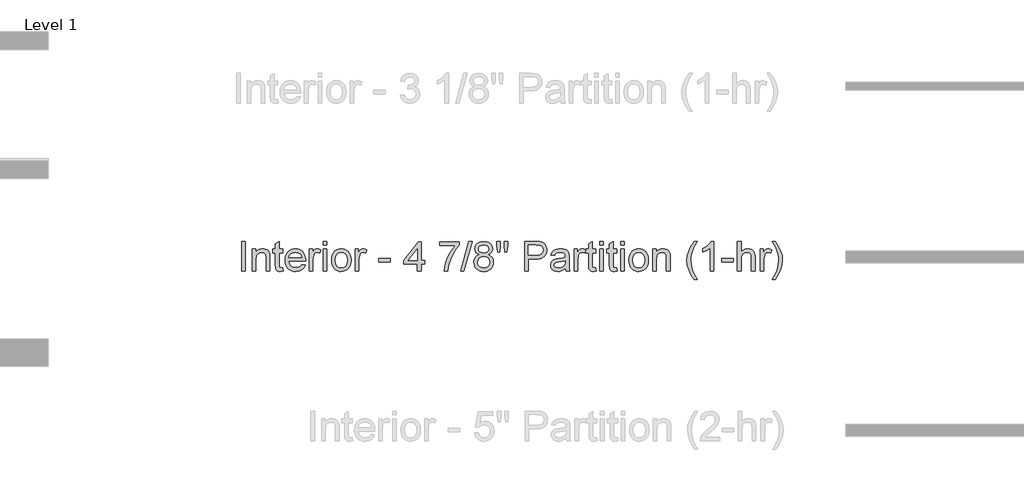
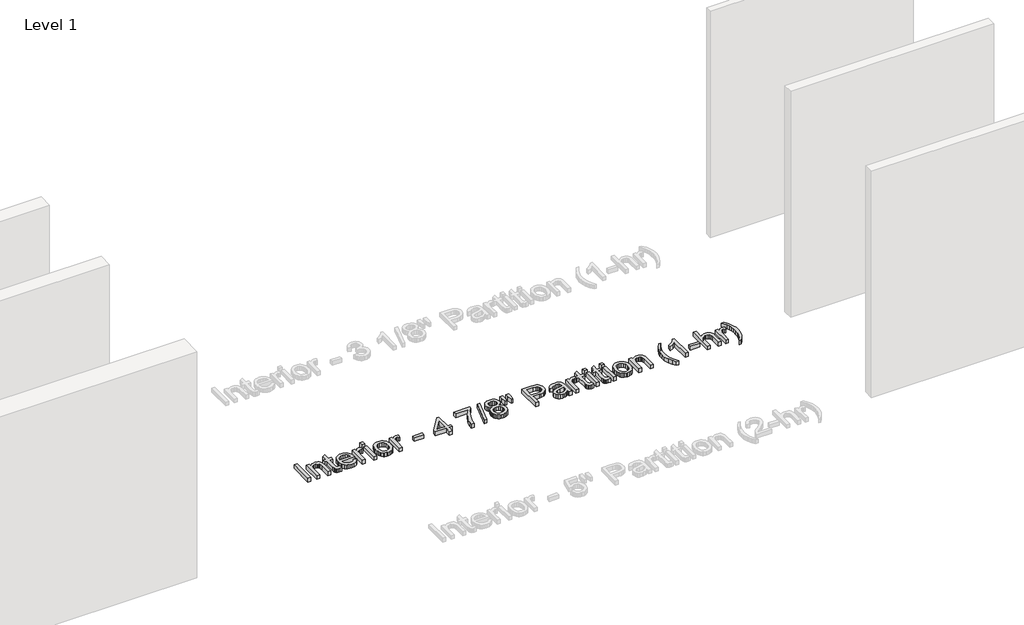
# One storey, part 35 of 42: 1 proxy.
"""IFC4 building model written with IfcOpenShell, lengths in millimetres."""

from ifc_helpers import new_model, si_unit, origin, origin_with_axes, place, context, project, spatial, polyline, outline, extrude, element, save

model = new_model("IFC4")

# Units and contexts
model_context = context("Model", 3, world=origin())
ifc_project = project(units=[si_unit("LENGTHUNIT", "METRE", prefix="MILLI")], contexts=[model_context])

# Site, building, storey
site = spatial("IfcSite", under=ifc_project)
building = spatial("IfcBuilding", under=site)
storey = spatial("IfcBuildingStorey", under=building, Name="Level 1", Elevation=0.0)

# Proxy
placement = place(None, origin())
element("IfcBuildingElementProxy", 1, Name="8\" Arial", ObjectType="8\" Arial", at=placement, inside=storey, context=model_context, shape_type="SweptSolid", body=[
    extrude(outline(polyline([(5292.0577476, 13738.6052202), (5292.0577476, 14043.1723143), (5330.1286344, 14043.1723143), (5330.1286344, 13738.6052202), (5292.0577476, 13738.6052202)])), origin_with_axes(), (0.0, 0.0, 1.0), 50.8),
    extrude(outline(polyline([(5401.511547, 13738.6052202), (5401.511547, 13962.2716799), (5439.5824338, 13962.2716799), (5439.5824338, 13931.0416556), (5452.8087209, 13946.7867928), (5468.6932779, 13958.0333195), (5487.2361048, 13964.7812354), (5508.4372016, 13967.0305407), (5527.2031002, 13965.218084), (5544.3889082, 13959.7807137), (5558.7212586, 13951.3969393), (5568.9267844, 13940.7452703), (5580.3406147, 13912.7497842), (5582.3482591, 13875.9429699), (5582.3482591, 13738.6052202), (5544.2773724, 13738.6052202), (5544.2773724, 13870.812323), (5539.8902975, 13904.4961349), (5533.820891, 13914.5250624), (5524.3868212, 13922.3046845), (5512.2944814, 13927.2959116), (5498.2502651, 13928.959654), (5475.9523996, 13925.2232046), (5456.9448402, 13914.0138566), (5449.3487874, 13904.8632736), (5443.9230354, 13892.3573219), (5439.5824338, 13857.2793125), (5439.5824338, 13738.6052202), (5401.511547, 13738.6052202)])), origin_with_axes(), (0.0, 0.0, 1.0), 50.8),
    extrude(outline(polyline([(5715.5963628, 13770.3557449), (5720.3552236, 13737.4898622), (5691.8764158, 13733.8463593), (5673.6031337, 13735.4264499), (5659.9771767, 13740.1667214), (5650.3479192, 13747.4723164), (5644.0647357, 13756.7483772), (5640.6071259, 13772.6794074), (5639.4545893, 13799.9499108), (5639.4545893, 13924.2007931), (5610.9014242, 13924.2007931), (5610.9014242, 13962.2716799), (5639.4545893, 13962.2716799), (5639.4545893, 14016.6267936), (5677.525476, 14039.008311), (5677.525476, 13962.2716799), (5715.5963628, 13962.2716799), (5715.5963628, 13924.2007931), (5677.525476, 13924.2007931), (5677.525476, 13801.0652688), (5679.5331204, 13781.4349678), (5686.0393755, 13774.4825695), (5699.014707, 13771.9172461), (5715.5963628, 13770.3557449)])), origin_with_axes(), (0.0, 0.0, 1.0), 50.8),
    extrude(outline(polyline([(5910.2635142, 13805.229272), (5947.590829, 13800.4704112), (5934.1414703, 13772.3448), (5912.6801232, 13751.3203015), (5883.6901096, 13738.2148449), (5847.6547512, 13733.8463593), (5824.032398, 13735.7308496), (5802.9846629, 13741.3843206), (5784.5115459, 13750.8067721), (5768.6130469, 13763.9982042), (5755.8282557, 13780.5914783), (5746.696262, 13800.2194556), (5741.2170658, 13822.8821362), (5739.390667, 13848.57952), (5741.2356551, 13875.1482773), (5746.7706192, 13898.5661482), (5755.9955594, 13918.8331327), (5768.9104757, 13935.9492308), (5784.7671487, 13949.5473039), (5802.8173592, 13959.2602133), (5823.0611071, 13965.0879589), (5845.4983924, 13967.0305407), (5867.2130187, 13965.0926062), (5886.8502907, 13959.2788026), (5904.4102083, 13949.5891298), (5919.8927717, 13936.023588), (5932.5311722, 13918.9446685), (5941.5586011, 13898.7148626), (5946.9750584, 13875.3341703), (5948.7805442, 13848.8025916), (5948.5574726, 13838.5412979), (5777.4615538, 13838.5412979), (5784.0514607, 13810.0439008), (5799.3597494, 13789.0937595), (5821.4531326, 13776.2113744), (5848.3983232, 13771.9172461), (5868.6606604, 13773.9063012), (5885.725638, 13779.8734666), (5899.5932559, 13790.1905282), (5910.2635142, 13805.229272)]), holes=[polyline([(5777.4615538, 13876.6121847), (5910.7096574, 13876.6121847), (5905.5604213, 13896.7258075), (5895.4664313, 13911.1139258), (5873.2708069, 13924.4982219), (5845.349678, 13928.959654), (5819.6871491, 13925.399803), (5798.467463, 13914.72025), (5783.7168533, 13898.0735317), (5777.4615538, 13876.6121847)])]), origin_with_axes(), (0.0, 0.0, 1.0), 50.8),
    extrude(outline(polyline([(5986.8514309, 13738.6052202), (5986.8514309, 13962.2716799), (6020.1634569, 13962.2716799), (6020.1634569, 13929.1827256), (6032.4695736, 13948.3668834), (6043.8090467, 13959.6691779), (6055.1856984, 13965.1902), (6067.6033509, 13967.0305407), (6086.5644371, 13964.0934313), (6105.8229521, 13955.282103), (6093.1078707, 13921.1521479), (6079.7235746, 13927.0077775), (6066.3392785, 13928.959654), (6054.9719214, 13927.0821347), (6044.8128689, 13921.4495767), (6036.6056929, 13912.489534), (6031.0939654, 13900.6295605), (6026.4652296, 13879.3634011), (6024.9223177, 13856.1639545), (6024.9223177, 13738.6052202), (5986.8514309, 13738.6052202)])), origin_with_axes(), (0.0, 0.0, 1.0), 50.8),
    extrude(outline(polyline([(6129.6172563, 14005.1014275), (6129.6172563, 14043.1723143), (6167.688143, 14043.1723143), (6167.688143, 14005.1014275), (6129.6172563, 14005.1014275)])), origin_with_axes(), (0.0, 0.0, 1.0), 50.8),
    extrude(outline(polyline([(6129.6172563, 13738.6052202), (6129.6172563, 13962.2716799), (6167.688143, 13962.2716799), (6167.688143, 13738.6052202), (6129.6172563, 13738.6052202)])), origin_with_axes(), (0.0, 0.0, 1.0), 50.8),
    extrude(outline(polyline([(6215.2767515, 13850.43845), (6217.3355165, 13879.405227), (6223.5118115, 13904.3660098), (6233.8056364, 13925.3207985), (6248.2169914, 13942.2695929), (6262.7259402, 13953.1025076), (6278.7406223, 13960.8403038), (6296.2610377, 13965.4829815), (6315.2871864, 13967.0305407), (6336.290772, 13965.1460504), (6355.2820658, 13959.4925795), (6372.2610678, 13950.070128), (6387.2277781, 13936.8786959), (6399.443272, 13920.3644263), (6408.1686248, 13900.9734626), (6413.4038364, 13878.7058046), (6415.148907, 13853.5614525), (6412.0630831, 13815.1001904), (6402.8056117, 13785.8220426), (6387.6460374, 13763.8959631), (6366.8539051, 13747.4909057), (6342.1580198, 13737.2574959), (6315.2871864, 13733.8463593), (6293.9768774, 13735.7238787), (6274.8089853, 13741.3564366), (6257.78351, 13750.7440332), (6242.9004516, 13763.8866684), (6230.8150828, 13780.5612707), (6222.1826765, 13800.5447684), (6217.0032327, 13823.8371615), (6215.2767515, 13850.43845)]), holes=[polyline([(6253.3476383, 13850.5128072), (6257.7533024, 13816.0575394), (6270.9702948, 13791.5103685), (6290.860846, 13776.8155267), (6315.2871864, 13771.9172461), (6339.6019911, 13776.8434106), (6359.4553637, 13791.6219043), (6372.6723561, 13816.4943879), (6377.0780202, 13851.7025224), (6372.6444721, 13885.1539681), (6359.3438279, 13909.3665316), (6339.4625713, 13924.0613734), (6315.2871864, 13928.959654), (6290.860846, 13924.0799627), (6270.9702948, 13909.4408888), (6257.7533024, 13884.9494858), (6253.3476383, 13850.5128072)])]), origin_with_axes(), (0.0, 0.0, 1.0), 50.8),
    extrude(outline(polyline([(6457.9786546, 13738.6052202), (6457.9786546, 13962.2716799), (6491.2906805, 13962.2716799), (6491.2906805, 13929.1827256), (6503.5967972, 13948.3668834), (6514.9362703, 13959.6691779), (6526.312922, 13965.1902), (6538.7305745, 13967.0305407), (6557.6916607, 13964.0934313), (6576.9501757, 13955.282103), (6564.2350944, 13921.1521479), (6550.8507983, 13927.0077775), (6537.4665021, 13928.959654), (6526.0991451, 13927.0821347), (6515.9400925, 13921.4495767), (6507.7329165, 13912.489534), (6502.221189, 13900.6295605), (6497.5924533, 13879.3634011), (6496.0495413, 13856.1639545), (6496.0495413, 13738.6052202), (6457.9786546, 13738.6052202)])), origin_with_axes(), (0.0, 0.0, 1.0), 50.8),
    extrude(outline(polyline([(6700.6805577, 13829.0235762), (6700.6805577, 13867.094463), (6819.6520788, 13867.094463), (6819.6520788, 13829.0235762), (6700.6805577, 13829.0235762)])), origin_with_axes(), (0.0, 0.0, 1.0), 50.8),
    extrude(outline(polyline([(7095.6660078, 13738.6052202), (7095.6660078, 13809.9881329), (6957.6590433, 13809.9881329), (6957.6590433, 13848.0590196), (7105.1837295, 14038.4134534), (7133.7368945, 14038.4134534), (7133.7368945, 13848.0590196), (7171.8077813, 13848.0590196), (7171.8077813, 13809.9881329), (7133.7368945, 13809.9881329), (7133.7368945, 13738.6052202), (7095.6660078, 13738.6052202)]), holes=[polyline([(7095.6660078, 13848.0590196), (7095.6660078, 13965.6921111), (7004.5040797, 13848.0590196), (7095.6660078, 13848.0590196)])]), origin_with_axes(), (0.0, 0.0, 1.0), 50.8),
    extrude(outline(polyline([(7324.0913283, 14000.3425666), (7324.0913283, 14038.4134534), (7523.9634838, 14038.4134534), (7523.9634838, 14007.6295723), (7495.4753813, 13971.5756246), (7467.2661183, 13925.7251157), (7442.38434, 13874.2606382), (7423.8786917, 13821.3647846), (7414.8071132, 13781.7881645), (7409.7508235, 13738.6052202), (7371.6799368, 13738.6052202), (7375.7974668, 13777.8472329), (7386.8116271, 13824.487787), (7404.424989, 13873.9260308), (7428.3401237, 13921.5611125), (7456.2612526, 13964.6232264), (7485.8925971, 14000.3425666), (7324.0913283, 14000.3425666)])), origin_with_axes(), (0.0, 0.0, 1.0), 50.8),
    extrude(outline(polyline([(7538.2400664, 13738.6052202), (7623.8995616, 14043.1723143), (7658.2525883, 14043.1723143), (7572.5930931, 13738.6052202), (7538.2400664, 13738.6052202)])), origin_with_axes(), (0.0, 0.0, 1.0), 50.8),
    extrude(outline(polyline([(7731.7175026, 13906.355065), (7711.3343349, 13916.3932871), (7697.0298684, 13930.0006548), (7688.5810315, 13946.8983286), (7685.7647525, 13966.8074691), (7687.2983698, 13982.3341821), (7691.8992216, 13996.5689387), (7699.5673079, 14009.511739), (7710.3026288, 14021.1625828), (7723.5893311, 14030.7918403), (7738.9115617, 14037.6698814), (7775.6626082, 14043.1723143), (7812.6367262, 14037.5397563), (7828.1262606, 14030.4990589), (7841.6174452, 14020.6420824), (7852.5479537, 14008.7635196), (7860.3554598, 13995.658063), (7865.0399634, 13981.3257126), (7866.6014646, 13965.7664683), (7863.8223643, 13946.4986587), (7855.4850631, 13929.889119), (7841.4966148, 13916.3654031), (7821.7640726, 13906.355065), (7845.1958855, 13894.2813145), (7862.2515684, 13876.5006489), (7872.6522819, 13853.8681759), (7876.1191863, 13827.2390034), (7874.3996761, 13808.2500333), (7869.2411453, 13790.8411537), (7860.6435939, 13775.0123646), (7848.6070221, 13760.763666), (7833.7634659, 13748.9873443), (7816.7449616, 13740.575686), (7797.5515091, 13735.528691), (7776.1831086, 13733.8463593), (7754.814708, 13735.535662), (7735.6212556, 13740.60357), (7718.6027513, 13749.0500832), (7703.7591951, 13760.8752018), (7691.7226232, 13775.2238179), (7683.1250719, 13791.2408236), (7677.9665411, 13808.9262191), (7676.2470309, 13828.2800042), (7679.8533551, 13855.9408829), (7690.6723278, 13878.6941863), (7708.14627, 13895.7591639), (7731.7175026, 13906.355065)]), holes=[polyline([(7723.8356393, 13965.6921111), (7727.2095973, 13949.0732768), (7737.3314712, 13935.8005164), (7753.9038323, 13927.100724), (7776.6292518, 13924.2007931), (7798.8248762, 13927.0821347), (7815.1462818, 13935.7261592), (7825.1845039, 13948.5527764), (7828.5305779, 13963.9818955), (7825.0729681, 13979.9965776), (7814.7001386, 13993.241454), (7798.1556614, 14002.1364341), (7776.1831086, 14005.1014275), (7754.071136, 14002.2014967), (7737.5545428, 13993.5017042), (7727.2653652, 13980.7494443), (7723.8356393, 13965.6921111)]), polyline([(7714.3179176, 13829.6184338), (7715.9073028, 13815.0537172), (7720.6754583, 13800.953733), (7729.4774919, 13788.6569109), (7743.1685115, 13779.5016806), (7759.5642742, 13773.8133547), (7776.4805374, 13771.9172461), (7802.3940218, 13775.904651), (7821.8384298, 13787.8668656), (7833.9958321, 13805.9821387), (7838.0482996, 13828.4287186), (7833.865707, 13851.2563792), (7821.3179294, 13869.7713222), (7801.4273782, 13882.0402603), (7775.216465, 13886.1299064), (7749.6654719, 13882.0960282), (7730.4162516, 13869.9943938), (7718.3425011, 13851.8326476), (7714.3179176, 13829.6184338)])]), origin_with_axes(), (0.0, 0.0, 1.0), 50.8),
    extrude(outline(polyline([(7918.7258623, 13933.7185148), (7909.4312122, 13992.5350606), (7909.4312122, 14043.1723143), (7947.502099, 14043.1723143), (7947.502099, 13992.5350606), (7939.1740925, 13933.7185148), (7918.7258623, 13933.7185148)])), origin_with_axes(), (0.0, 0.0, 1.0), 50.8),
    extrude(outline(polyline([(7994.6445643, 13933.7185148), (7985.5729858, 13992.5350606), (7985.5729858, 14043.1723143), (8023.6438725, 14043.1723143), (8023.6438725, 13992.5350606), (8014.7210084, 13933.7185148), (7994.6445643, 13933.7185148)])), origin_with_axes(), (0.0, 0.0, 1.0), 50.8),
    extrude(outline(polyline([(8194.9628629, 13738.6052202), (8194.9628629, 14043.1723143), (8307.8370936, 14043.1723143), (8353.3437004, 14040.2723834), (8373.6339216, 14034.8536024), (8390.3364078, 14026.0329795), (8403.7857665, 14013.4108447), (8414.316605, 13996.587528), (8421.1202889, 13976.7434501), (8423.3881835, 13955.0590314), (8421.8568899, 13936.3628428), (8417.2630091, 13919.1630928), (8409.6065411, 13903.4597815), (8398.8874859, 13889.2529088), (8384.1717311, 13877.4765871), (8364.5251645, 13869.0649288), (8339.947786, 13864.0179338), (8310.4395956, 13862.3356021), (8233.0337497, 13862.3356021), (8233.0337497, 13738.6052202), (8194.9628629, 13738.6052202)]), holes=[polyline([(8233.0337497, 13900.4064889), (8312.6703116, 13900.4064889), (8346.4284808, 13903.9012773), (8368.735641, 13914.3856426), (8381.1718828, 13931.2089593), (8385.3172967, 13953.7206018), (8382.8728038, 13970.822758), (8375.5393248, 13985.2480549), (8364.2277357, 13996.1042062), (8349.848912, 14002.4989255), (8311.7780252, 14005.1014275), (8233.0337497, 14005.1014275), (8233.0337497, 13900.4064889)])]), origin_with_axes(), (0.0, 0.0, 1.0), 50.8),
    extrude(outline(polyline([(8613.7426173, 13767.1583853), (8595.5529871, 13751.5619624), (8576.8242671, 13741.3564366), (8557.1289036, 13735.7238787), (8536.0393426, 13733.8463593), (8504.2237553, 13738.3635593), (8480.7547638, 13751.9151591), (8466.2829936, 13772.4935144), (8461.4590702, 13798.0909807), (8463.2808217, 13813.8732966), (8468.7460759, 13828.205647), (8477.1763235, 13840.4745851), (8487.8930551, 13850.066664), (8514.5501115, 13862.5586738), (8547.4903515, 13868.2841782), (8586.416346, 13874.3071115), (8613.5195457, 13881.3710455), (8613.7426173, 13889.8477664), (8611.121526, 13906.8383868), (8603.258252, 13917.9547883), (8585.672774, 13926.2084376), (8561.1720764, 13928.959654), (8538.4931302, 13927.1286079), (8522.6550464, 13921.6354697), (8511.854663, 13911.4764172), (8504.2888179, 13895.6476281), (8466.2179311, 13900.4064889), (8472.8264273, 13921.2265051), (8482.688051, 13937.5850893), (8496.7229727, 13950.0956883), (8515.8513626, 13959.3717491), (8539.2459968, 13965.1158428), (8566.0796516, 13967.0305407), (8591.8165377, 13965.3389144), (8612.2182947, 13960.2640355), (8627.6009406, 13952.6331277), (8638.2804935, 13943.2734151), (8645.3630169, 13931.7015758), (8649.954574, 13917.4342879), (8651.813504, 13884.122262), (8651.813504, 13836.7567251), (8653.7467913, 13770.6159951), (8661.3312257, 13738.6052202), (8623.260339, 13738.6052202), (8617.1630485, 13751.8408019), (8613.7426173, 13767.1583853)]), holes=[polyline([(8613.7426173, 13843.3001588), (8552.3235695, 13831.6260783), (8519.5692226, 13825.4544306), (8504.7349611, 13815.4162085), (8499.529957, 13800.76784), (8502.3648253, 13789.4469562), (8510.8694301, 13780.1708954), (8524.8578785, 13773.9806584), (8544.1442774, 13771.9172461), (8564.5925076, 13774.1944354), (8582.6613074, 13781.0260032), (8597.3096759, 13791.0921092), (8607.4966124, 13803.0729132), (8612.0138124, 13815.4162085), (8613.5195457, 13832.5183647), (8613.7426173, 13843.3001588)])]), origin_with_axes(), (0.0, 0.0, 1.0), 50.8),
    extrude(outline(polyline([(8704.1609733, 13738.6052202), (8704.1609733, 13962.2716799), (8737.4729992, 13962.2716799), (8737.4729992, 13929.1827256), (8749.779116, 13948.3668834), (8761.1185891, 13959.6691779), (8772.4952408, 13965.1902), (8784.9128933, 13967.0305407), (8803.8739795, 13964.0934313), (8823.1324945, 13955.282103), (8810.4174131, 13921.1521479), (8797.033117, 13927.0077775), (8783.6488209, 13928.959654), (8772.2814638, 13927.0821347), (8762.1224113, 13921.4495767), (8753.9152353, 13912.489534), (8748.4035078, 13900.6295605), (8743.774772, 13879.3634011), (8742.2318601, 13856.1639545), (8742.2318601, 13738.6052202), (8704.1609733, 13738.6052202)])), origin_with_axes(), (0.0, 0.0, 1.0), 50.8),
    extrude(outline(polyline([(8927.827433, 13770.3557449), (8932.5862939, 13737.4898622), (8904.107486, 13733.8463593), (8885.8342039, 13735.4264499), (8872.2082469, 13740.1667214), (8862.5789894, 13747.4723164), (8856.295806, 13756.7483772), (8852.8381961, 13772.6794074), (8851.6856595, 13799.9499108), (8851.6856595, 13924.2007931), (8823.1324945, 13924.2007931), (8823.1324945, 13962.2716799), (8851.6856595, 13962.2716799), (8851.6856595, 14016.6267936), (8889.7565463, 14039.008311), (8889.7565463, 13962.2716799), (8927.827433, 13962.2716799), (8927.827433, 13924.2007931), (8889.7565463, 13924.2007931), (8889.7565463, 13801.0652688), (8891.7641907, 13781.4349678), (8898.2704458, 13774.4825695), (8911.2457773, 13771.9172461), (8927.827433, 13770.3557449)])), origin_with_axes(), (0.0, 0.0, 1.0), 50.8),
    extrude(outline(polyline([(8965.8983198, 13738.6052202), (8965.8983198, 13962.2716799), (9003.9692066, 13962.2716799), (9003.9692066, 13738.6052202), (8965.8983198, 13738.6052202)])), origin_with_axes(), (0.0, 0.0, 1.0), 50.8),
    extrude(outline(polyline([(8965.8983198, 14005.1014275), (8965.8983198, 14043.1723143), (9003.9692066, 14043.1723143), (9003.9692066, 14005.1014275), (8965.8983198, 14005.1014275)])), origin_with_axes(), (0.0, 0.0, 1.0), 50.8),
    extrude(outline(polyline([(9141.9761711, 13770.3557449), (9146.7350319, 13737.4898622), (9118.256224, 13733.8463593), (9099.982942, 13735.4264499), (9086.3569849, 13740.1667214), (9076.7277274, 13747.4723164), (9070.444544, 13756.7483772), (9066.9869342, 13772.6794074), (9065.8343975, 13799.9499108), (9065.8343975, 13924.2007931), (9037.2812325, 13924.2007931), (9037.2812325, 13962.2716799), (9065.8343975, 13962.2716799), (9065.8343975, 14016.6267936), (9103.9052843, 14039.008311), (9103.9052843, 13962.2716799), (9141.9761711, 13962.2716799), (9141.9761711, 13924.2007931), (9103.9052843, 13924.2007931), (9103.9052843, 13801.0652688), (9105.9129287, 13781.4349678), (9112.4191838, 13774.4825695), (9125.3945153, 13771.9172461), (9141.9761711, 13770.3557449)])), origin_with_axes(), (0.0, 0.0, 1.0), 50.8),
    extrude(outline(polyline([(9180.0470578, 14005.1014275), (9180.0470578, 14043.1723143), (9218.1179446, 14043.1723143), (9218.1179446, 14005.1014275), (9180.0470578, 14005.1014275)])), origin_with_axes(), (0.0, 0.0, 1.0), 50.8),
    extrude(outline(polyline([(9180.0470578, 13738.6052202), (9180.0470578, 13962.2716799), (9218.1179446, 13962.2716799), (9218.1179446, 13738.6052202), (9180.0470578, 13738.6052202)])), origin_with_axes(), (0.0, 0.0, 1.0), 50.8),
    extrude(outline(polyline([(9265.706553, 13850.43845), (9267.765318, 13879.405227), (9273.941613, 13904.3660098), (9284.235438, 13925.3207985), (9298.6467929, 13942.2695929), (9313.1557417, 13953.1025076), (9329.1704238, 13960.8403038), (9346.6908392, 13965.4829815), (9365.716988, 13967.0305407), (9386.7205735, 13965.1460504), (9405.7118673, 13959.4925795), (9422.6908693, 13950.070128), (9437.6575796, 13936.8786959), (9449.8730735, 13920.3644263), (9458.5984263, 13900.9734626), (9463.833638, 13878.7058046), (9465.5787085, 13853.5614525), (9462.4928847, 13815.1001904), (9453.2354132, 13785.8220426), (9438.0758389, 13763.8959631), (9417.2837066, 13747.4909057), (9392.5878214, 13737.2574959), (9365.716988, 13733.8463593), (9344.406679, 13735.7238787), (9325.2387868, 13741.3564366), (9308.2133115, 13750.7440332), (9293.3302531, 13763.8866684), (9281.2448843, 13780.5612707), (9272.612478, 13800.5447684), (9267.4330343, 13823.8371615), (9265.706553, 13850.43845)]), holes=[polyline([(9303.7774398, 13850.5128072), (9308.1831039, 13816.0575394), (9321.4000963, 13791.5103685), (9341.2906475, 13776.8155267), (9365.716988, 13771.9172461), (9390.0317926, 13776.8434106), (9409.8851652, 13791.6219043), (9423.1021576, 13816.4943879), (9427.5078217, 13851.7025224), (9423.0742737, 13885.1539681), (9409.7736294, 13909.3665316), (9389.8923728, 13924.0613734), (9365.716988, 13928.959654), (9341.2906475, 13924.0799627), (9321.4000963, 13909.4408888), (9308.1831039, 13884.9494858), (9303.7774398, 13850.5128072)])]), origin_with_axes(), (0.0, 0.0, 1.0), 50.8),
    extrude(outline(polyline([(9508.4084561, 13738.6052202), (9508.4084561, 13962.2716799), (9546.4793429, 13962.2716799), (9546.4793429, 13931.0416556), (9559.7056299, 13946.7867928), (9575.5901869, 13958.0333195), (9594.1330139, 13964.7812354), (9615.3341107, 13967.0305407), (9634.1000092, 13965.218084), (9651.2858173, 13959.7807137), (9665.6181677, 13951.3969393), (9675.8236935, 13940.7452703), (9687.2375238, 13912.7497842), (9689.2451682, 13875.9429699), (9689.2451682, 13738.6052202), (9651.1742815, 13738.6052202), (9651.1742815, 13870.812323), (9646.7872066, 13904.4961349), (9640.7178001, 13914.5250624), (9631.2837303, 13922.3046845), (9619.1913905, 13927.2959116), (9605.1471742, 13928.959654), (9582.8493087, 13925.2232046), (9563.8417492, 13914.0138566), (9556.2456964, 13904.8632736), (9550.8199445, 13892.3573219), (9546.4793429, 13857.2793125), (9546.4793429, 13738.6052202), (9508.4084561, 13738.6052202)])), origin_with_axes(), (0.0, 0.0, 1.0), 50.8),
    extrude(outline(polyline([(9936.7059321, 13652.945725), (9907.2047128, 13694.3440965), (9882.6482472, 13742.248723), (9866.0851808, 13794.3359421), (9860.5641586, 13848.2820912), (9864.6909833, 13895.5918602), (9877.0714572, 13940.8568061), (9901.646512, 13992.126096), (9936.7059321, 14043.1723143), (9965.2590972, 14043.1723143), (9929.6419981, 13982.8686245), (9908.2271243, 13924.4238647), (9901.0330651, 13886.3343887), (9898.6350454, 13848.0590196), (9902.7990486, 13799.252812), (9915.2910583, 13750.4651937), (9936.1110745, 13701.6961647), (9965.2590972, 13652.945725), (9936.7059321, 13652.945725)])), origin_with_axes(), (0.0, 0.0, 1.0), 50.8),
    extrude(outline(polyline([(10136.5780876, 13738.6052202), (10098.5072009, 13738.6052202), (10098.5072009, 13975.9534048), (10062.4439585, 13950.262992), (10022.3654273, 13931.0416556), (10022.3654273, 13967.0305407), (10052.2663167, 13983.2961784), (10078.1705065, 14002.6476399), (10098.5908527, 14023.2259952), (10112.0402114, 14043.1723143), (10136.5780876, 14043.1723143), (10136.5780876, 13738.6052202)])), origin_with_axes(), (0.0, 0.0, 1.0), 50.8),
    extrude(outline(polyline([(10217.478722, 13829.0235762), (10217.478722, 13867.094463), (10336.4502431, 13867.094463), (10336.4502431, 13829.0235762), (10217.478722, 13829.0235762)])), origin_with_axes(), (0.0, 0.0, 1.0), 50.8),
    extrude(outline(polyline([(10379.2799907, 13738.6052202), (10379.2799907, 14043.1723143), (10417.3508775, 14043.1723143), (10417.3508775, 13931.19037), (10431.3346785, 13946.8704447), (10447.0379898, 13958.0704981), (10464.4608114, 13964.7905301), (10483.6031433, 13967.0305407), (10506.5981076, 13964.5860478), (10526.3585337, 13957.2525688), (10541.9177779, 13945.6063723), (10552.3091967, 13930.2237264), (10558.1648263, 13909.0876921), (10560.1167028, 13880.1813303), (10560.1167028, 13738.6052202), (10522.0458161, 13738.6052202), (10522.0458161, 13876.2403987), (10519.0157601, 13900.0718815), (10509.9255923, 13916.3932871), (10495.2772238, 13925.8180622), (10475.5725656, 13928.959654), (10459.4835263, 13926.8404738), (10444.3797199, 13920.4829331), (10431.8691209, 13910.5004789), (10423.5597037, 13897.5065581), (10418.903084, 13880.2370982), (10417.3508775, 13857.4280269), (10417.3508775, 13738.6052202), (10379.2799907, 13738.6052202)])), origin_with_axes(), (0.0, 0.0, 1.0), 50.8),
    extrude(outline(polyline([(10612.4641721, 13738.6052202), (10612.4641721, 13962.2716799), (10645.776198, 13962.2716799), (10645.776198, 13929.1827256), (10658.0823147, 13948.3668834), (10669.4217878, 13959.6691779), (10680.7984395, 13965.1902), (10693.2160921, 13967.0305407), (10712.1771782, 13964.0934313), (10731.4356932, 13955.282103), (10718.7206119, 13921.1521479), (10705.3363158, 13927.0077775), (10691.9520197, 13928.959654), (10680.5846626, 13927.0821347), (10670.4256101, 13921.4495767), (10662.218434, 13912.489534), (10656.7067065, 13900.6295605), (10652.0779708, 13879.3634011), (10650.5350589, 13856.1639545), (10650.5350589, 13738.6052202), (10612.4641721, 13738.6052202)])), origin_with_axes(), (0.0, 0.0, 1.0), 50.8),
    extrude(outline(polyline([(10764.7477191, 13652.945725), (10736.1945541, 13652.945725), (10765.3425767, 13701.6961647), (10786.1625929, 13750.4651937), (10798.6546027, 13799.252812), (10802.8186059, 13848.0590196), (10800.4205862, 13886.0555492), (10793.226527, 13923.7546499), (10784.1363592, 13953.6276553), (10772.0347248, 13982.2737669), (10736.1945541, 14043.1723143), (10764.7477191, 14043.1723143), (10799.8071393, 13992.126096), (10824.3821941, 13940.8568061), (10836.762668, 13895.5918602), (10840.8894927, 13848.2820912), (10835.3405866, 13794.3359421), (10818.6938682, 13742.248723), (10794.1095188, 13694.3440965), (10764.7477191, 13652.945725)])), origin_with_axes(), (0.0, 0.0, 1.0), 50.8),
])

save(model, "model.ifc")

# Revit data of these elements
# Element 1 (IfcBuildingElementProxy, "8\" Arial")
#   Phase Created = New Construction
